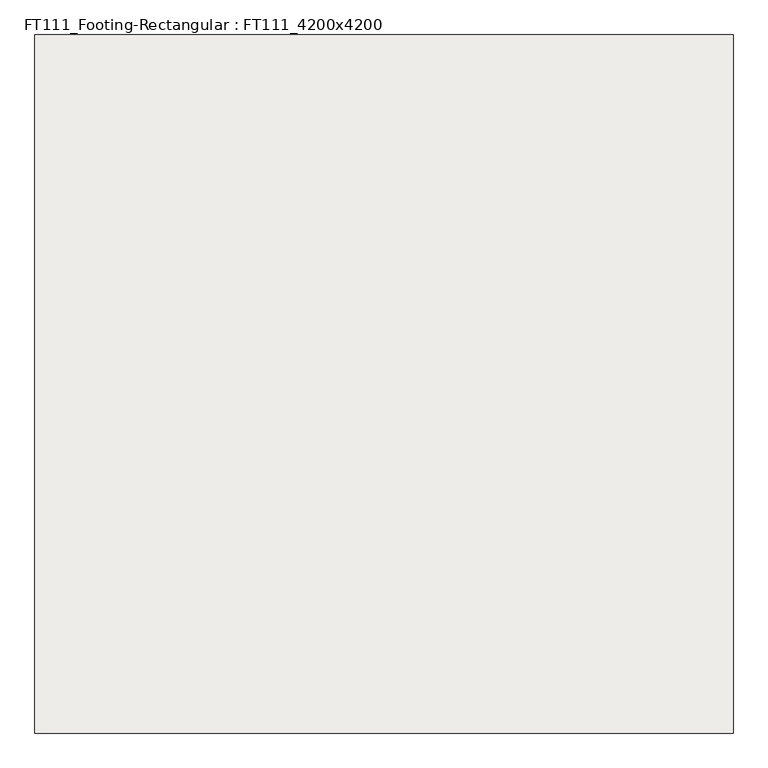
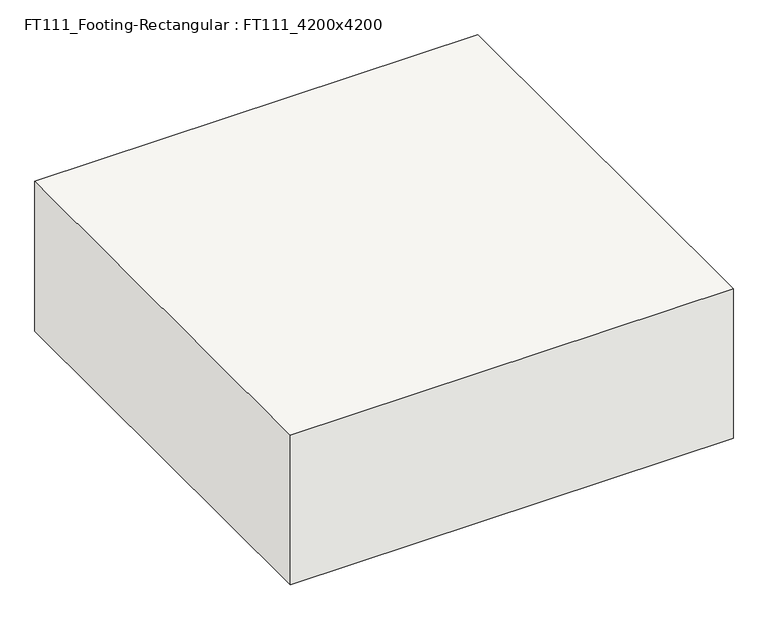
"""IFC4 building model written with IfcOpenShell, lengths in millimetres: slab geometry, FT111_Footing-Rectangular : FT111_4200x4200."""

from ifc_helpers import new_model, si_unit, origin, origin_with_axes, place, context, project, spatial, polyline, outline, extrude, source, transform, mapped, element, save


def ft111_footing_rectangular_ft111_4200x4200_1dfe1a53(model_context):
    return source(origin(), model_context, "Body", "SweptSolid", [
        extrude(outline(polyline([(2100.0, 2100.0), (2100.0, -2100.0), (-2100.0, -2100.0), (-2100.0, 2100.0), (2100.0, 2100.0)])), origin_with_axes(), (0.0, 0.0, 1.0), 1500.0),
    ])


if __name__ == "__main__":
    model = new_model("IFC4")
    model_context = context("Model", 3, world=origin())
    ifc_project = project(units=[si_unit("LENGTHUNIT", "METRE", prefix="MILLI")], contexts=[model_context])
    site = spatial("IfcSite", under=ifc_project)
    building = spatial("IfcBuilding", under=site)
    placement = place(None, origin())
    ft111_footing_rectangular_ft111_4200x4200_shape = ft111_footing_rectangular_ft111_4200x4200_1dfe1a53(model_context)
    element("IfcSlab", 1, ObjectType="FT111_Footing-Rectangular : FT111_4200x4200", at=placement, inside=building, context=model_context, shape_type="MappedRepresentation", body=[
        mapped(ft111_footing_rectangular_ft111_4200x4200_shape, transform((0.0, 0.0, 0.0), x_axis=(1.0, 0.0, 0.0), y_axis=(0.0, 1.0, 0.0), z_axis=(0.0, 0.0, 1.0))),
    ])
    save(model, "model.ifc")

# Revit data of these elements
# Type "FT111_Footing-Rectangular : FT111_4200x4200"
#   Assembly Code = "A1010100"
#   Width = 4200 mm
#   Length = 4200 mm
#   Foundation Thickness = 1500 mm
#   Structural Material [instance default] = Concrete, Cast-in-Place gray
# Element 1 (IfcSlab, "FT111_Footing-Rectangular : FT111_4200x4200")
#   Materials on its faces: "Concrete, Cast-in-Place gray"
# Materials
#   "Concrete, Cast-in-Place gray": class "Concrete", colour RGB 192 192 192, transparency 0, Description = "Cast-in-place concrete", Cost = 0
